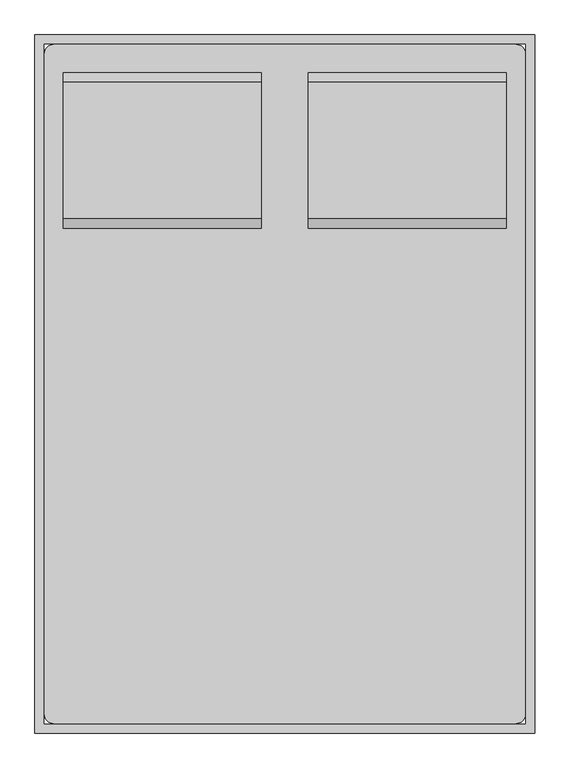
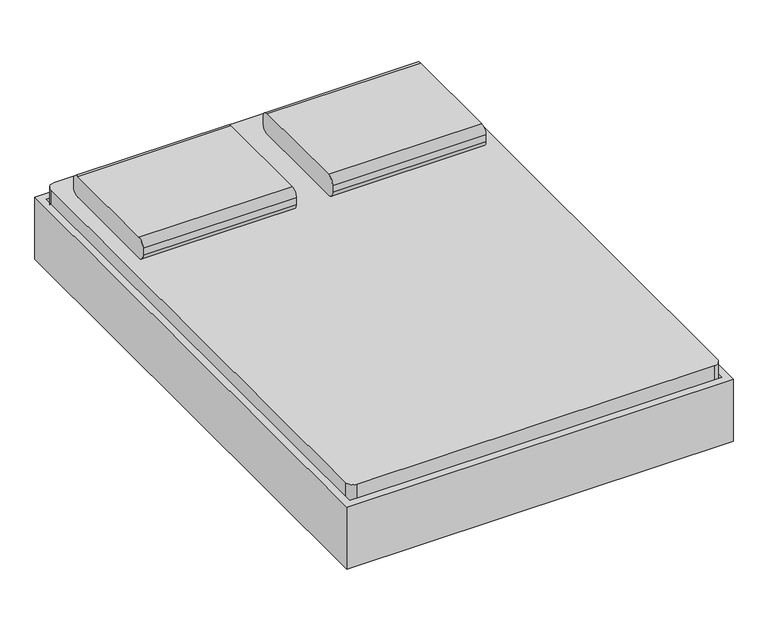
"""IFC4 building model written with IfcOpenShell, lengths in millimetres: furniture geometry, Cama-Caixa : 1346 x 1880 mm - Casal."""

from ifc_helpers import new_model, si_unit, point, frame, frame_2d, origin, place, context, project, spatial, polyline, circle_curve, trimmed, segment, composite_curve, outline, extrude, source, transform, mapped, element, save
from ifc_brep_helpers import plane_surface, cylinder_surface, revolved_surface, advanced_brep


def furniture_b32eb57e(model_context):
    return source(origin(), model_context, "Body", "SolidModel", [
        extrude(outline(composite_curve([segment(polyline([(578.5704918, 406.4), (210.2704918, 406.4)]), True, "CONTINUOUS"), segment(trimmed(circle_curve(frame_2d((210.2704918, 431.8)), 25.4), [point((210.2704918, 406.4))], [point((184.8704918, 431.8))], False, "CARTESIAN"), True, "CONTINUOUS"), segment(polyline([(184.8704918, 431.8), (184.8704918, 457.2)]), True, "CONTINUOUS"), segment(trimmed(circle_curve(frame_2d((210.2704918, 457.2)), 25.4), [point((184.8704918, 457.2))], [point((210.2704918, 482.6))], False, "CARTESIAN"), True, "CONTINUOUS"), segment(polyline([(210.2704918, 482.6), (578.5704918, 482.6)]), True, "CONTINUOUS"), segment(trimmed(circle_curve(frame_2d((578.5704918, 457.2)), 25.4), [point((578.5704918, 482.6))], [point((603.9704918, 457.2))], False, "CARTESIAN"), True, "CONTINUOUS"), segment(polyline([(603.9704918, 457.2), (603.9704918, 431.8)]), True, "CONTINUOUS"), segment(trimmed(circle_curve(frame_2d((578.5704918, 431.8)), 25.4), [point((603.9704918, 431.8))], [point((578.5704918, 406.4))], False, "CARTESIAN"), True, "CONTINUOUS")], self_intersect=False)), frame((402.652459, 0.0, 0.0), z_axis=(1.0, 0.0, 0.0), x_axis=(0.0, 1.0, 0.0)), (0.0, 0.0, 1.0), 533.3),
        extrude(outline(composite_curve([segment(polyline([(578.5704918, 406.4), (210.2704918, 406.4)]), True, "CONTINUOUS"), segment(trimmed(circle_curve(frame_2d((210.2704918, 431.8)), 25.4), [point((210.2704918, 406.4))], [point((184.8704918, 431.8))], False, "CARTESIAN"), True, "CONTINUOUS"), segment(polyline([(184.8704918, 431.8), (184.8704918, 457.2)]), True, "CONTINUOUS"), segment(trimmed(circle_curve(frame_2d((210.2704918, 457.2)), 25.4), [point((184.8704918, 457.2))], [point((210.2704918, 482.6))], False, "CARTESIAN"), True, "CONTINUOUS"), segment(polyline([(210.2704918, 482.6), (578.5704918, 482.6)]), True, "CONTINUOUS"), segment(trimmed(circle_curve(frame_2d((578.5704918, 457.2)), 25.4), [point((578.5704918, 482.6))], [point((603.9704918, 457.2))], False, "CARTESIAN"), True, "CONTINUOUS"), segment(polyline([(603.9704918, 457.2), (603.9704918, 431.8)]), True, "CONTINUOUS"), segment(trimmed(circle_curve(frame_2d((578.5704918, 431.8)), 25.4), [point((603.9704918, 431.8))], [point((578.5704918, 406.4))], False, "CARTESIAN"), True, "CONTINUOUS")], self_intersect=False)), frame((-257.647541, 0.0, 0.0), z_axis=(1.0, 0.0, 0.0), x_axis=(0.0, 1.0, 0.0)), (0.0, 0.0, 1.0), 533.3),
        advanced_brep(
        [(-308.1231784, 451.5704918, 177.8), (-308.1231784, 375.3704918, 177.8), (-308.1231784, 375.3704918, 196.85), (-308.1231784, 451.5704918, 196.85), (-257.3231784, 451.5704918, 177.8), (-257.3231784, 375.3704918, 177.8), (-245.1869899, 375.3704918, 196.85), (-245.1869899, 451.5704918, 196.85), (-181.2523099, 451.5704918, 14.6654962), (-181.2523099, 375.3704918, 14.6654962), (-163.9871466, 375.3704918, 22.716374), (-163.9871466, 451.5704918, 22.716374), (-158.2320921, 375.3704918, 0.0), (-158.2320921, 451.5704918, 0.0), (-158.2320921, 375.3704918, 19.05), (-158.2320921, 451.5704918, 19.05), (-79.6195862, 451.5704918, 0.0), (-79.6195862, 375.3704918, 0.0), (-79.6195862, 375.3704918, 19.05), (-79.6195862, 451.5704918, 19.05), (-66.9195862, 375.3704918, 3.4029547), (-66.9195862, 451.5704918, 3.4029547), (-76.4445862, 375.3704918, 19.9007387), (-76.4445862, 451.5704918, 19.9007387), (-6.822541, 451.5704918, 38.1), (-6.822541, 375.3704918, 38.1), (-11.9269731, 375.3704918, 57.15), (-11.9269731, 451.5704918, 57.15), (685.4518216, 451.5704918, 38.1), (685.4518216, 375.3704918, 38.1), (690.5562537, 375.3704918, 57.15), (690.5562537, 451.5704918, 57.15), (745.5488669, 451.5704918, 3.4029547), (745.5488669, 375.3704918, 3.4029547), (755.0738669, 375.3704918, 19.9007387), (755.0738669, 451.5704918, 19.9007387), (758.2488669, 375.3704918, 0.0), (758.2488669, 451.5704918, 0.0), (758.2488669, 375.3704918, 19.05), (758.2488669, 451.5704918, 19.05), (836.8613728, 451.5704918, 0.0), (836.8613728, 375.3704918, 0.0), (836.8613728, 375.3704918, 19.05), (836.8613728, 451.5704918, 19.05), (859.8815906, 375.3704918, 14.6654962), (859.8815906, 451.5704918, 14.6654962), (842.6164272, 375.3704918, 22.716374), (842.6164272, 451.5704918, 22.716374), (935.952459, 451.5704918, 177.8), (935.952459, 375.3704918, 177.8), (923.8162705, 375.3704918, 196.85), (923.8162705, 451.5704918, 196.85), (986.752459, 451.5704918, 177.8), (986.752459, 451.5704918, 196.85), (986.752459, 375.3704918, 196.85), (986.752459, 375.3704918, 177.8)],
        [
            (0, 1),
            (1, 2),
            (2, 3),
            (3, 0),
            (0, 4),
            (4, 5),
            (5, 1),
            (5, 6),
            (6, 2),
            (6, 7),
            (7, 3),
            (7, 4),
            (4, 8),
            (8, 9),
            (9, 5),
            (9, 10),
            (10, 6),
            (10, 11),
            (11, 7),
            (11, 8),
            (12, 9, circle_curve(frame((-158.2320921, 375.3704918, 25.4), z_axis=(0.0, 1.0, 0.0), x_axis=(-0.906307787036649, 0.0, -0.4226182617407015)), 25.4)),
            (8, 13, circle_curve(frame((-158.2320921, 451.5704918, 25.4), z_axis=(0.0, -1.0, 0.0), x_axis=(-0.906307787036649, 0.0, -0.4226182617407015)), 25.4)),
            (13, 12),
            (14, 10, circle_curve(frame((-158.2320921, 375.3704918, 25.4), z_axis=(0.0, 1.0, 0.0), x_axis=(-0.906307787036649, 0.0, -0.4226182617407015)), 6.35)),
            (12, 14),
            (15, 11, circle_curve(frame((-158.2320921, 451.5704918, 25.4), z_axis=(0.0, 1.0, 0.0), x_axis=(-0.906307787036649, 0.0, -0.4226182617407015)), 6.35)),
            (14, 15),
            (15, 13),
            (13, 16),
            (16, 17),
            (17, 12),
            (17, 18),
            (18, 14),
            (18, 19),
            (19, 15),
            (19, 16),
            (20, 17, circle_curve(frame((-79.6195862, 375.3704918, 25.4), z_axis=(0.0, 1.0, 0.0), x_axis=(0.0, 0.0, -1.0)), 25.4)),
            (16, 21, circle_curve(frame((-79.6195862, 451.5704918, 25.4), z_axis=(0.0, -1.0, 0.0), x_axis=(0.0, 0.0, -1.0)), 25.4)),
            (21, 20),
            (22, 18, circle_curve(frame((-79.6195862, 375.3704918, 25.4), z_axis=(0.0, 1.0, 0.0), x_axis=(0.0, 0.0, -1.0)), 6.35)),
            (20, 22),
            (23, 19, circle_curve(frame((-79.6195862, 451.5704918, 25.4), z_axis=(0.0, 1.0, 0.0), x_axis=(0.0, 0.0, -1.0)), 6.35)),
            (22, 23),
            (23, 21),
            (21, 24),
            (24, 25),
            (25, 20),
            (25, 26),
            (26, 22),
            (26, 27),
            (27, 23),
            (27, 24),
            (24, 28),
            (28, 29),
            (29, 25),
            (29, 30),
            (30, 26),
            (30, 31),
            (31, 27),
            (31, 28),
            (28, 32),
            (32, 33),
            (33, 29),
            (33, 34),
            (34, 30),
            (34, 35),
            (35, 31),
            (35, 32),
            (36, 33, circle_curve(frame((758.2488669, 375.3704918, 25.4), z_axis=(0.0, 1.0, 0.0), x_axis=(-0.5000000000000463, 0.0, -0.8660254037844118)), 25.4)),
            (32, 37, circle_curve(frame((758.2488669, 451.5704918, 25.4), z_axis=(0.0, -1.0, 0.0), x_axis=(-0.5000000000000463, 0.0, -0.8660254037844118)), 25.4)),
            (37, 36),
            (38, 34, circle_curve(frame((758.2488669, 375.3704918, 25.4), z_axis=(0.0, 1.0, 0.0), x_axis=(-0.5000000000000463, 0.0, -0.8660254037844118)), 6.35)),
            (36, 38),
            (39, 35, circle_curve(frame((758.2488669, 451.5704918, 25.4), z_axis=(0.0, 1.0, 0.0), x_axis=(-0.5000000000000463, 0.0, -0.8660254037844118)), 6.35)),
            (38, 39),
            (39, 37),
            (37, 40),
            (40, 41),
            (41, 36),
            (41, 42),
            (42, 38),
            (42, 43),
            (43, 39),
            (43, 40),
            (44, 41, circle_curve(frame((836.8613728, 375.3704918, 25.4), z_axis=(0.0, 1.0, 0.0), x_axis=(0.0, 0.0, -1.0)), 25.4)),
            (40, 45, circle_curve(frame((836.8613728, 451.5704918, 25.4), z_axis=(0.0, -1.0, 0.0), x_axis=(0.0, 0.0, -1.0)), 25.4)),
            (45, 44),
            (46, 42, circle_curve(frame((836.8613728, 375.3704918, 25.4), z_axis=(0.0, 1.0, 0.0), x_axis=(0.0, 0.0, -1.0)), 6.35)),
            (44, 46),
            (47, 43, circle_curve(frame((836.8613728, 451.5704918, 25.4), z_axis=(0.0, 1.0, 0.0), x_axis=(0.0, 0.0, -1.0)), 6.35)),
            (46, 47),
            (47, 45),
            (45, 48),
            (48, 49),
            (49, 44),
            (49, 50),
            (50, 46),
            (50, 51),
            (51, 47),
            (51, 48),
            (52, 53),
            (53, 54),
            (54, 55),
            (55, 52),
            (48, 52),
            (55, 49),
            (54, 50),
            (53, 51),
        ],
        [
            plane_surface(frame((-308.1231784, 705.5704918, -152.9490627), z_axis=(-1.0, 0.0, 0.0), x_axis=(0.0, 1.0, 0.0))),
            plane_surface(frame((-308.1231784, 451.5704918, 177.8), z_axis=(0.0, 0.0, -1.0), x_axis=(1.0, 0.0, 0.0))),
            plane_surface(frame((-308.1231784, 375.3704918, 177.8), z_axis=(0.0, -1.0, 0.0), x_axis=(1.0, 0.0, 0.0))),
            plane_surface(frame((-308.1231784, 375.3704918, 196.85), z_axis=(0.0, 0.0, 1.0), x_axis=(1.0, 0.0, 0.0))),
            plane_surface(frame((-308.1231784, 451.5704918, 196.85), z_axis=(0.0, 1.0, 0.0), x_axis=(1.0, 0.0, 0.0))),
            plane_surface(frame((-257.3231784, 451.5704918, 177.8), z_axis=(-0.9063077870366486, 0.0, -0.4226182617407026), x_axis=(0.4226182617407026, 0.0, -0.9063077870366486))),
            plane_surface(frame((-257.3231784, 375.3704918, 177.8), z_axis=(0.0, -1.0000000000000002, 0.0), x_axis=(0.4226182617407026, 0.0, -0.9063077870366486))),
            plane_surface(frame((-245.1869899, 375.3704918, 196.85), z_axis=(0.9063077870366487, 0.0, 0.4226182617407023), x_axis=(0.4226182617407023, 0.0, -0.9063077870366487))),
            plane_surface(frame((-245.1869899, 451.5704918, 196.85), z_axis=(0.0, 1.0, 0.0), x_axis=(0.4226182617407027, 0.0, -0.9063077870366485))),
            cylinder_surface(frame((-158.2320921, 705.5704918, 25.4), z_axis=(0.0, -1.0, 0.0), x_axis=(-0.906307787036649, 0.0, -0.4226182617407015)), 25.4),
            plane_surface(frame((-158.2320921, 375.3704918, 25.4), z_axis=(0.0, -1.0, 0.0), x_axis=(-0.906307787036649, 0.0, -0.4226182617407015))),
            revolved_surface(polyline([(-163.9871465476827, 375.3704918, 22.716374037946544), (-163.9871465476827, 451.5704918, 22.716374037946544)]), (-158.2320921, 705.5704918, 25.4), (0.0, -1.0, 0.0)),
            plane_surface(frame((-158.2320921, 451.5704918, 25.4), z_axis=(0.0, 1.0, 0.0), x_axis=(-0.906307787036649, 0.0, -0.4226182617407015))),
            plane_surface(frame((-158.2320921, 451.5704918, 0.0), z_axis=(0.0, 0.0, -1.0), x_axis=(1.0, 0.0, 0.0))),
            plane_surface(frame((-158.2320921, 375.3704918, 0.0), z_axis=(0.0, -1.0, 0.0), x_axis=(1.0, 0.0, 0.0))),
            plane_surface(frame((-158.2320921, 375.3704918, 19.05), z_axis=(0.0, 0.0, 1.0), x_axis=(1.0, 0.0, 0.0))),
            plane_surface(frame((-158.2320921, 451.5704918, 19.05), z_axis=(0.0, 1.0, 0.0), x_axis=(1.0, 0.0, 0.0))),
            cylinder_surface(frame((-79.6195862, 705.5704918, 25.4), z_axis=(0.0, -1.0, 0.0), x_axis=(0.0, 0.0, -1.0)), 25.4),
            plane_surface(frame((-79.6195862, 375.3704918, 25.4), z_axis=(0.0, -1.0, 0.0), x_axis=(0.0, 0.0, -1.0))),
            revolved_surface(polyline([(-79.6195862, 375.3704918, 19.049999999999997), (-79.6195862, 451.5704918, 19.049999999999997)]), (-79.6195862, 705.5704918, 25.4), (0.0, -1.0, 0.0)),
            plane_surface(frame((-79.6195862, 451.5704918, 25.4), z_axis=(0.0, 1.0, 0.0), x_axis=(0.0, 0.0, -1.0))),
            plane_surface(frame((-66.9195862, 451.5704918, 3.4029547), z_axis=(0.4999999999998744, 0.0, -0.8660254037845112), x_axis=(0.8660254037845112, 0.0, 0.4999999999998744))),
            plane_surface(frame((-66.9195862, 375.3704918, 3.4029547), z_axis=(0.0, -1.0000000000000002, 0.0), x_axis=(0.8660254037845112, 0.0, 0.4999999999998745))),
            plane_surface(frame((-76.4445862, 375.3704918, 19.9007387), z_axis=(-0.4999999999998741, 0.0, 0.8660254037845113), x_axis=(0.8660254037845113, 0.0, 0.4999999999998741))),
            plane_surface(frame((-76.4445862, 451.5704918, 19.9007387), z_axis=(0.0, 1.0, 0.0), x_axis=(0.866025403784511, 0.0, 0.49999999999987477))),
            plane_surface(frame((-6.822541, 451.5704918, 38.1), z_axis=(0.0, 0.0, -1.0), x_axis=(1.0, 0.0, 0.0))),
            plane_surface(frame((-6.822541, 375.3704918, 38.1), z_axis=(0.0, -1.0, 0.0), x_axis=(1.0, 0.0, 0.0))),
            plane_surface(frame((-11.9269731, 375.3704918, 57.15), z_axis=(0.0, 0.0, 1.0), x_axis=(1.0, 0.0, 0.0))),
            plane_surface(frame((-11.9269731, 451.5704918, 57.15), z_axis=(0.0, 1.0, 0.0), x_axis=(1.0, 0.0, 0.0))),
            plane_surface(frame((685.4518216, 451.5704918, 38.1), z_axis=(-0.5000000000000494, 0.0, -0.8660254037844102), x_axis=(0.8660254037844102, 0.0, -0.5000000000000494))),
            plane_surface(frame((685.4518216, 375.3704918, 38.1), z_axis=(0.0, -1.0, 0.0), x_axis=(0.8660254037844112, 0.0, -0.5000000000000476))),
            plane_surface(frame((690.5562537, 375.3704918, 57.15), z_axis=(0.5000000000000488, 0.0, 0.8660254037844105), x_axis=(0.8660254037844105, 0.0, -0.5000000000000488))),
            plane_surface(frame((690.5562537, 451.5704918, 57.15), z_axis=(0.0, 1.0, 0.0), x_axis=(0.8660254037844106, 0.0, -0.5000000000000485))),
            cylinder_surface(frame((758.2488669, 705.5704918, 25.4), z_axis=(0.0, -1.0, 0.0), x_axis=(-0.5000000000000463, 0.0, -0.8660254037844118)), 25.4),
            plane_surface(frame((758.2488669, 375.3704918, 25.4), z_axis=(0.0, -1.0000000000000002, 0.0), x_axis=(-0.5000000000000464, 0.0, -0.866025403784412))),
            revolved_surface(polyline([(755.0738668999998, 375.3704918, 19.90073868596898), (755.0738668999998, 451.5704918, 19.90073868596898)]), (758.2488669, 705.5704918, 25.4), (0.0, -1.0, 0.0)),
            plane_surface(frame((758.2488669, 451.5704918, 25.4), z_axis=(0.0, 1.0000000000000002, 0.0), x_axis=(-0.5000000000000464, 0.0, -0.866025403784412))),
            plane_surface(frame((758.2488669, 451.5704918, 0.0), z_axis=(0.0, 0.0, -1.0), x_axis=(1.0, 0.0, 0.0))),
            plane_surface(frame((758.2488669, 375.3704918, 0.0), z_axis=(0.0, -1.0, 0.0), x_axis=(1.0, 0.0, 0.0))),
            plane_surface(frame((758.2488669, 375.3704918, 19.05), z_axis=(0.0, 0.0, 1.0), x_axis=(1.0, 0.0, 0.0))),
            plane_surface(frame((758.2488669, 451.5704918, 19.05), z_axis=(0.0, 1.0, 0.0), x_axis=(1.0, 0.0, 0.0))),
            cylinder_surface(frame((836.8613728, 705.5704918, 25.4), z_axis=(0.0, -1.0, 0.0), x_axis=(0.0, 0.0, -1.0)), 25.4),
            plane_surface(frame((836.8613728, 375.3704918, 25.4), z_axis=(0.0, -1.0, 0.0), x_axis=(0.0, 0.0, -1.0))),
            revolved_surface(polyline([(836.8613728, 375.3704918, 19.049999999999997), (836.8613728, 451.5704918, 19.049999999999997)]), (836.8613728, 705.5704918, 25.4), (0.0, -1.0, 0.0)),
            plane_surface(frame((836.8613728, 451.5704918, 25.4), z_axis=(0.0, 1.0, 0.0), x_axis=(0.0, 0.0, -1.0))),
            plane_surface(frame((859.8815906, 451.5704918, 14.6654962), z_axis=(0.90630778703668, 0.0, -0.422618261740635), x_axis=(0.422618261740635, 0.0, 0.90630778703668))),
            plane_surface(frame((859.8815906, 375.3704918, 14.6654962), z_axis=(0.0, -1.0000000000000002, 0.0), x_axis=(0.4226182617406349, 0.0, 0.9063077870366801))),
            plane_surface(frame((842.6164272, 375.3704918, 22.716374), z_axis=(-0.9063077870366805, 0.0, 0.4226182617406341), x_axis=(0.4226182617406341, 0.0, 0.9063077870366805))),
            plane_surface(frame((842.6164272, 451.5704918, 22.716374), z_axis=(0.0, 1.0, 0.0), x_axis=(0.42261826174063455, 0.0, 0.9063077870366802))),
            plane_surface(frame((986.752459, 705.5704918, -152.9490627), z_axis=(1.0, 0.0, 0.0), x_axis=(0.0, 1.0, 0.0))),
            plane_surface(frame((935.952459, 451.5704918, 177.8), z_axis=(0.0, 0.0, -1.0), x_axis=(1.0, 0.0, 0.0))),
            plane_surface(frame((935.952459, 375.3704918, 177.8), z_axis=(0.0, -1.0, 0.0), x_axis=(1.0, 0.0, 0.0))),
            plane_surface(frame((923.8162705, 375.3704918, 196.85), z_axis=(0.0, 0.0, 1.0), x_axis=(1.0, 0.0, 0.0))),
            plane_surface(frame((923.8162705, 451.5704918, 196.85), z_axis=(0.0, 1.0, 0.0), x_axis=(1.0, 0.0, 0.0))),
        ],
        [
            (0, [[1, 2, 3, 4]]),
            (1, [[-1, 5, 6, 7]]),
            (2, [[-2, -7, 8, 9]]),
            (3, [[-3, -9, 10, 11]]),
            (4, [[-4, -11, 12, -5]]),
            (5, [[-6, 13, 14, 15]]),
            (6, [[-8, -15, 16, 17]]),
            (7, [[-10, -17, 18, 19]]),
            (8, [[-12, -19, 20, -13]]),
            (9, [[21, -14, 22, 23]]),
            (10, [[24, -16, -21, 25]]),
            (11, [[26, -18, -24, 27]]),
            (12, [[-22, -20, -26, 28]]),
            (13, [[-23, 29, 30, 31]]),
            (14, [[-25, -31, 32, 33]]),
            (15, [[-27, -33, 34, 35]]),
            (16, [[-28, -35, 36, -29]]),
            (17, [[37, -30, 38, 39]]),
            (18, [[40, -32, -37, 41]]),
            (19, [[42, -34, -40, 43]]),
            (20, [[-38, -36, -42, 44]]),
            (21, [[-39, 45, 46, 47]]),
            (22, [[-41, -47, 48, 49]]),
            (23, [[-43, -49, 50, 51]]),
            (24, [[-44, -51, 52, -45]]),
            (25, [[-46, 53, 54, 55]]),
            (26, [[-48, -55, 56, 57]]),
            (27, [[-50, -57, 58, 59]]),
            (28, [[-52, -59, 60, -53]]),
            (29, [[-54, 61, 62, 63]]),
            (30, [[-56, -63, 64, 65]]),
            (31, [[-58, -65, 66, 67]]),
            (32, [[-60, -67, 68, -61]]),
            (33, [[69, -62, 70, 71]]),
            (34, [[72, -64, -69, 73]]),
            (35, [[74, -66, -72, 75]]),
            (36, [[-70, -68, -74, 76]]),
            (37, [[-71, 77, 78, 79]]),
            (38, [[-73, -79, 80, 81]]),
            (39, [[-75, -81, 82, 83]]),
            (40, [[-76, -83, 84, -77]]),
            (41, [[85, -78, 86, 87]]),
            (42, [[88, -80, -85, 89]]),
            (43, [[90, -82, -88, 91]]),
            (44, [[-86, -84, -90, 92]]),
            (45, [[-87, 93, 94, 95]]),
            (46, [[-89, -95, 96, 97]]),
            (47, [[-91, -97, 98, 99]]),
            (48, [[-92, -99, 100, -93]]),
            (49, [[101, 102, 103, 104]]),
            (50, [[-94, 105, -104, 106]]),
            (51, [[-96, -106, -103, 107]]),
            (52, [[-98, -107, -102, 108]]),
            (53, [[-100, -108, -101, -105]]),
        ],
    ),
        extrude(outline(composite_curve([segment(polyline([(-283.047541, 680.1704918), (961.352459, 680.1704918)]), True, "CONTINUOUS"), segment(trimmed(circle_curve(frame_2d((961.352459, 654.7704918)), 25.4), [point((961.352459, 680.1704918))], [point((986.752459, 654.7704918))], False, "CARTESIAN"), True, "CONTINUOUS"), segment(polyline([(986.752459, 654.7704918), (986.752459, -1123.6295082)]), True, "CONTINUOUS"), segment(trimmed(circle_curve(frame_2d((961.352459, -1123.6295082)), 25.4), [point((986.752459, -1123.6295082))], [point((961.352459, -1149.0295082))], False, "CARTESIAN"), True, "CONTINUOUS"), segment(polyline([(961.352459, -1149.0295082), (-283.047541, -1149.0295082)]), True, "CONTINUOUS"), segment(trimmed(circle_curve(frame_2d((-283.047541, -1123.6295082)), 25.4), [point((-283.047541, -1149.0295082))], [point((-308.447541, -1123.6295082))], False, "CARTESIAN"), True, "CONTINUOUS"), segment(polyline([(-308.447541, -1123.6295082), (-308.447541, 654.7704918)]), True, "CONTINUOUS"), segment(trimmed(circle_curve(frame_2d((-283.047541, 654.7704918)), 25.4), [point((-308.447541, 654.7704918))], [point((-283.047541, 680.1704918))], False, "CARTESIAN"), True, "CONTINUOUS")], self_intersect=False)), frame((0.0, 0.0, 203.2), z_axis=(0.0, 0.0, 1.0), x_axis=(1.0, 0.0, 0.0)), (0.0, 0.0, 1.0), 203.2),
        advanced_brep(
        [(-308.447541, -869.6295082, 196.85), (-308.447541, -869.6295082, 177.8), (-308.447541, -945.8295082, 177.8), (-308.447541, -945.8295082, 196.85), (-245.5113525, -869.6295082, 196.85), (-257.647541, -869.6295082, 177.8), (-257.647541, -945.8295082, 177.8), (-245.5113525, -945.8295082, 196.85), (-164.3115092, -869.6295082, 22.716374), (-181.5766725, -869.6295082, 14.6654962), (-181.5766725, -945.8295082, 14.6654962), (-164.3115092, -945.8295082, 22.716374), (-158.5564547, -869.6295082, 0.0), (-158.5564547, -869.6295082, 19.05), (-158.5564547, -945.8295082, 0.0), (-158.5564547, -945.8295082, 19.05), (-79.9439489, -869.6295082, 19.05), (-79.9439489, -869.6295082, 0.0), (-79.9439489, -945.8295082, 0.0), (-79.9439489, -945.8295082, 19.05), (-67.2439489, -869.6295082, 3.4029547), (-76.7689489, -869.6295082, 19.9007387), (-67.2439489, -945.8295082, 3.4029547), (-76.7689489, -945.8295082, 19.9007387), (-12.2513357, -869.6295082, 57.15), (-7.1469036, -869.6295082, 38.1), (-7.1469036, -945.8295082, 38.1), (-12.2513357, -945.8295082, 57.15), (690.5562537, -869.6295082, 57.15), (685.4518216, -869.6295082, 38.1), (685.4518216, -945.8295082, 38.1), (690.5562537, -945.8295082, 57.15), (755.0738669, -869.6295082, 19.9007387), (745.5488669, -869.6295082, 3.4029547), (745.5488669, -945.8295082, 3.4029547), (755.0738669, -945.8295082, 19.9007387), (758.2488669, -869.6295082, 0.0), (758.2488669, -869.6295082, 19.05), (758.2488669, -945.8295082, 0.0), (758.2488669, -945.8295082, 19.05), (836.8613728, -869.6295082, 19.05), (836.8613728, -869.6295082, 0.0), (836.8613728, -945.8295082, 0.0), (836.8613728, -945.8295082, 19.05), (859.8815906, -869.6295082, 14.6654962), (842.6164272, -869.6295082, 22.716374), (859.8815906, -945.8295082, 14.6654962), (842.6164272, -945.8295082, 22.716374), (923.8162705, -869.6295082, 196.85), (935.952459, -869.6295082, 177.8), (935.952459, -945.8295082, 177.8), (923.8162705, -945.8295082, 196.85), (986.752459, -869.6295082, 196.85), (986.752459, -945.8295082, 196.85), (986.752459, -945.8295082, 177.8), (986.752459, -869.6295082, 177.8)],
        [
            (0, 1),
            (1, 2),
            (2, 3),
            (3, 0),
            (0, 4),
            (4, 5),
            (5, 1),
            (5, 6),
            (6, 2),
            (6, 7),
            (7, 3),
            (7, 4),
            (4, 8),
            (8, 9),
            (9, 5),
            (9, 10),
            (10, 6),
            (10, 11),
            (11, 7),
            (11, 8),
            (12, 9, circle_curve(frame((-158.5564547, -869.6295082, 25.4), z_axis=(0.0, 1.0, 0.0), x_axis=(-0.9063077870366625, 0.0, -0.4226182617406725)), 25.4)),
            (8, 13, circle_curve(frame((-158.5564547, -869.6295082, 25.4), z_axis=(0.0, -1.0, 0.0), x_axis=(-0.9063077870366625, 0.0, -0.4226182617406725)), 6.35)),
            (13, 12),
            (14, 10, circle_curve(frame((-158.5564547, -945.8295082, 25.4), z_axis=(0.0, 1.0, 0.0), x_axis=(-0.9063077870366625, 0.0, -0.4226182617406725)), 25.4)),
            (12, 14),
            (15, 11, circle_curve(frame((-158.5564547, -945.8295082, 25.4), z_axis=(0.0, 1.0, 0.0), x_axis=(-0.9063077870366625, 0.0, -0.4226182617406725)), 6.35)),
            (14, 15),
            (15, 13),
            (13, 16),
            (16, 17),
            (17, 12),
            (17, 18),
            (18, 14),
            (18, 19),
            (19, 15),
            (19, 16),
            (20, 17, circle_curve(frame((-79.9439489, -869.6295082, 25.4), z_axis=(0.0, 1.0, 0.0), x_axis=(0.0, 0.0, -1.0)), 25.4)),
            (16, 21, circle_curve(frame((-79.9439489, -869.6295082, 25.4), z_axis=(0.0, -1.0, 0.0), x_axis=(0.0, 0.0, -1.0)), 6.35)),
            (21, 20),
            (22, 18, circle_curve(frame((-79.9439489, -945.8295082, 25.4), z_axis=(0.0, 1.0, 0.0), x_axis=(0.0, 0.0, -1.0)), 25.4)),
            (20, 22),
            (23, 19, circle_curve(frame((-79.9439489, -945.8295082, 25.4), z_axis=(0.0, 1.0, 0.0), x_axis=(0.0, 0.0, -1.0)), 6.35)),
            (22, 23),
            (23, 21),
            (21, 24),
            (24, 25),
            (25, 20),
            (25, 26),
            (26, 22),
            (26, 27),
            (27, 23),
            (27, 24),
            (24, 28),
            (28, 29),
            (29, 25),
            (29, 30),
            (30, 26),
            (30, 31),
            (31, 27),
            (31, 28),
            (28, 32),
            (32, 33),
            (33, 29),
            (33, 34),
            (34, 30),
            (34, 35),
            (35, 31),
            (35, 32),
            (36, 33, circle_curve(frame((758.2488669, -869.6295082, 25.4), z_axis=(0.0, 1.0, 0.0), x_axis=(-0.5000000000000528, 0.0, -0.8660254037844081)), 25.4)),
            (32, 37, circle_curve(frame((758.2488669, -869.6295082, 25.4), z_axis=(0.0, -1.0, 0.0), x_axis=(-0.5000000000000528, 0.0, -0.8660254037844081)), 6.35)),
            (37, 36),
            (38, 34, circle_curve(frame((758.2488669, -945.8295082, 25.4), z_axis=(0.0, 1.0, 0.0), x_axis=(-0.5000000000000528, 0.0, -0.8660254037844081)), 25.4)),
            (36, 38),
            (39, 35, circle_curve(frame((758.2488669, -945.8295082, 25.4), z_axis=(0.0, 1.0, 0.0), x_axis=(-0.5000000000000528, 0.0, -0.8660254037844081)), 6.35)),
            (38, 39),
            (39, 37),
            (37, 40),
            (40, 41),
            (41, 36),
            (41, 42),
            (42, 38),
            (42, 43),
            (43, 39),
            (43, 40),
            (44, 41, circle_curve(frame((836.8613728, -869.6295082, 25.4), z_axis=(0.0, 1.0, 0.0), x_axis=(0.0, 0.0, -1.0)), 25.4)),
            (40, 45, circle_curve(frame((836.8613728, -869.6295082, 25.4), z_axis=(0.0, -1.0, 0.0), x_axis=(0.0, 0.0, -1.0)), 6.35)),
            (45, 44),
            (46, 42, circle_curve(frame((836.8613728, -945.8295082, 25.4), z_axis=(0.0, 1.0, 0.0), x_axis=(0.0, 0.0, -1.0)), 25.4)),
            (44, 46),
            (47, 43, circle_curve(frame((836.8613728, -945.8295082, 25.4), z_axis=(0.0, 1.0, 0.0), x_axis=(0.0, 0.0, -1.0)), 6.35)),
            (46, 47),
            (47, 45),
            (45, 48),
            (48, 49),
            (49, 44),
            (49, 50),
            (50, 46),
            (50, 51),
            (51, 47),
            (51, 48),
            (52, 53),
            (53, 54),
            (54, 55),
            (55, 52),
            (48, 52),
            (55, 49),
            (54, 50),
            (53, 51),
        ],
        [
            plane_surface(frame((-308.447541, -1174.4295082, -127.5947323), z_axis=(-1.0, 0.0, 0.0), x_axis=(0.0, 1.0, 0.0))),
            plane_surface(frame((-308.447541, -869.6295082, 196.85), z_axis=(0.0, 1.0, 0.0), x_axis=(1.0, 0.0, 0.0))),
            plane_surface(frame((-308.447541, -869.6295082, 177.8), z_axis=(0.0, 0.0, -1.0), x_axis=(1.0, 0.0, 0.0))),
            plane_surface(frame((-308.447541, -945.8295082, 177.8), z_axis=(0.0, -1.0, 0.0), x_axis=(1.0, 0.0, 0.0))),
            plane_surface(frame((-308.447541, -945.8295082, 196.85), z_axis=(0.0, 0.0, 1.0), x_axis=(1.0, 0.0, 0.0))),
            plane_surface(frame((-245.5113525, -869.6295082, 196.85), z_axis=(0.0, 1.0, 0.0), x_axis=(0.4226182617406714, 0.0, -0.906307787036663))),
            plane_surface(frame((-257.647541, -869.6295082, 177.8), z_axis=(-0.9063077870366631, 0.0, -0.42261826174067146), x_axis=(0.42261826174067146, 0.0, -0.9063077870366631))),
            plane_surface(frame((-257.647541, -945.8295082, 177.8), z_axis=(0.0, -1.0000000000000002, 0.0), x_axis=(0.4226182617406716, 0.0, -0.906307787036663))),
            plane_surface(frame((-245.5113525, -945.8295082, 196.85), z_axis=(0.906307787036663, 0.0, 0.4226182617406716), x_axis=(0.4226182617406716, 0.0, -0.906307787036663))),
            plane_surface(frame((-158.5564547, -869.6295082, 25.4), z_axis=(0.0, 1.0, 0.0), x_axis=(-0.9063077870366625, 0.0, -0.4226182617406725))),
            cylinder_surface(frame((-158.5564547, -1174.4295082, 25.4), z_axis=(0.0, -1.0, 0.0), x_axis=(-0.9063077870366625, 0.0, -0.4226182617406725)), 25.4),
            plane_surface(frame((-158.5564547, -945.8295082, 25.4), z_axis=(0.0, -1.0, 0.0), x_axis=(-0.9063077870366625, 0.0, -0.4226182617406725))),
            revolved_surface(polyline([(-164.31150914768278, -945.8295082, 22.71637403794673), (-164.31150914768278, -869.6295082, 22.71637403794673)]), (-158.5564547, -1174.4295082, 25.4), (0.0, -1.0, 0.0)),
            plane_surface(frame((-158.5564547, -869.6295082, 19.05), z_axis=(0.0, 1.0, 0.0), x_axis=(1.0, 0.0, 0.0))),
            plane_surface(frame((-158.5564547, -869.6295082, 0.0), z_axis=(0.0, 0.0, -1.0), x_axis=(1.0, 0.0, 0.0))),
            plane_surface(frame((-158.5564547, -945.8295082, 0.0), z_axis=(0.0, -1.0, 0.0), x_axis=(1.0, 0.0, 0.0))),
            plane_surface(frame((-158.5564547, -945.8295082, 19.05), z_axis=(0.0, 0.0, 1.0), x_axis=(1.0, 0.0, 0.0))),
            plane_surface(frame((-79.9439489, -869.6295082, 25.4), z_axis=(0.0, 1.0, 0.0), x_axis=(0.0, 0.0, -1.0))),
            cylinder_surface(frame((-79.9439489, -1174.4295082, 25.4), z_axis=(0.0, -1.0, 0.0), x_axis=(0.0, 0.0, -1.0)), 25.4),
            plane_surface(frame((-79.9439489, -945.8295082, 25.4), z_axis=(0.0, -1.0, 0.0), x_axis=(0.0, 0.0, -1.0))),
            revolved_surface(polyline([(-79.9439489, -945.8295082, 19.049999999999997), (-79.9439489, -869.6295082, 19.049999999999997)]), (-79.9439489, -1174.4295082, 25.4), (0.0, -1.0, 0.0)),
            plane_surface(frame((-76.7689489, -869.6295082, 19.9007387), z_axis=(0.0, 1.0000000000000002, 0.0), x_axis=(0.8660254037844788, 0.0, 0.49999999999993067))),
            plane_surface(frame((-67.2439489, -869.6295082, 3.4029547), z_axis=(0.49999999999993067, 0.0, -0.8660254037844787), x_axis=(0.8660254037844787, 0.0, 0.49999999999993067))),
            plane_surface(frame((-67.2439489, -945.8295082, 3.4029547), z_axis=(0.0, -1.0, 0.0), x_axis=(0.8660254037844782, 0.0, 0.4999999999999315))),
            plane_surface(frame((-76.7689489, -945.8295082, 19.9007387), z_axis=(-0.49999999999993044, 0.0, 0.8660254037844789), x_axis=(0.8660254037844789, 0.0, 0.49999999999993044))),
            plane_surface(frame((-12.2513357, -869.6295082, 57.15), z_axis=(0.0, 1.0, 0.0), x_axis=(1.0, 0.0, 0.0))),
            plane_surface(frame((-7.1469036, -869.6295082, 38.1), z_axis=(0.0, 0.0, -1.0), x_axis=(1.0, 0.0, 0.0))),
            plane_surface(frame((-7.1469036, -945.8295082, 38.1), z_axis=(0.0, -1.0, 0.0), x_axis=(1.0, 0.0, 0.0))),
            plane_surface(frame((-12.2513357, -945.8295082, 57.15), z_axis=(0.0, 0.0, 1.0), x_axis=(1.0, 0.0, 0.0))),
            plane_surface(frame((690.5562537, -869.6295082, 57.15), z_axis=(0.0, 1.0, 0.0), x_axis=(0.8660254037844087, 0.0, -0.5000000000000518))),
            plane_surface(frame((685.4518216, -869.6295082, 38.1), z_axis=(-0.5000000000000513, 0.0, -0.8660254037844092), x_axis=(0.8660254037844092, 0.0, -0.5000000000000513))),
            plane_surface(frame((685.4518216, -945.8295082, 38.1), z_axis=(0.0, -1.0, 0.0), x_axis=(0.8660254037844081, 0.0, -0.5000000000000531))),
            plane_surface(frame((690.5562537, -945.8295082, 57.15), z_axis=(0.5000000000000521, 0.0, 0.8660254037844086), x_axis=(0.8660254037844086, 0.0, -0.5000000000000521))),
            plane_surface(frame((758.2488669, -869.6295082, 25.4), z_axis=(0.0, 1.0000000000000002, 0.0), x_axis=(-0.500000000000053, 0.0, -0.8660254037844082))),
            cylinder_surface(frame((758.2488669, -1174.4295082, 25.4), z_axis=(0.0, -1.0, 0.0), x_axis=(-0.5000000000000528, 0.0, -0.8660254037844081)), 25.4),
            plane_surface(frame((758.2488669, -945.8295082, 25.4), z_axis=(0.0, -1.0000000000000002, 0.0), x_axis=(-0.500000000000053, 0.0, -0.8660254037844082))),
            revolved_surface(polyline([(755.0738668999998, -945.8295082, 19.900738685969007), (755.0738668999998, -869.6295082, 19.900738685969007)]), (758.2488669, -1174.4295082, 25.4), (0.0, -1.0, 0.0)),
            plane_surface(frame((758.2488669, -869.6295082, 19.05), z_axis=(0.0, 1.0, 0.0), x_axis=(1.0, 0.0, 0.0))),
            plane_surface(frame((758.2488669, -869.6295082, 0.0), z_axis=(0.0, 0.0, -1.0), x_axis=(1.0, 0.0, 0.0))),
            plane_surface(frame((758.2488669, -945.8295082, 0.0), z_axis=(0.0, -1.0, 0.0), x_axis=(1.0, 0.0, 0.0))),
            plane_surface(frame((758.2488669, -945.8295082, 19.05), z_axis=(0.0, 0.0, 1.0), x_axis=(1.0, 0.0, 0.0))),
            plane_surface(frame((836.8613728, -869.6295082, 25.4), z_axis=(0.0, 1.0, 0.0), x_axis=(0.0, 0.0, -1.0))),
            cylinder_surface(frame((836.8613728, -1174.4295082, 25.4), z_axis=(0.0, -1.0, 0.0), x_axis=(0.0, 0.0, -1.0)), 25.4),
            plane_surface(frame((836.8613728, -945.8295082, 25.4), z_axis=(0.0, -1.0, 0.0), x_axis=(0.0, 0.0, -1.0))),
            revolved_surface(polyline([(836.8613728, -945.8295082, 19.049999999999997), (836.8613728, -869.6295082, 19.049999999999997)]), (836.8613728, -1174.4295082, 25.4), (0.0, -1.0, 0.0)),
            plane_surface(frame((842.6164272, -869.6295082, 22.716374), z_axis=(0.0, 1.0, 0.0), x_axis=(0.4226182617405387, 0.0, 0.906307787036725))),
            plane_surface(frame((859.8815906, -869.6295082, 14.6654962), z_axis=(0.906307787036725, 0.0, -0.4226182617405386), x_axis=(0.4226182617405386, 0.0, 0.906307787036725))),
            plane_surface(frame((859.8815906, -945.8295082, 14.6654962), z_axis=(0.0, -1.0, 0.0), x_axis=(0.4226182617405387, 0.0, 0.906307787036725))),
            plane_surface(frame((842.6164272, -945.8295082, 22.716374), z_axis=(-0.9063077870367251, 0.0, 0.4226182617405384), x_axis=(0.4226182617405384, 0.0, 0.9063077870367251))),
            plane_surface(frame((986.752459, -1174.4295082, -127.5947323), z_axis=(1.0, 0.0, 0.0), x_axis=(0.0, 1.0, 0.0))),
            plane_surface(frame((923.8162705, -869.6295082, 196.85), z_axis=(0.0, 1.0, 0.0), x_axis=(1.0, 0.0, 0.0))),
            plane_surface(frame((935.952459, -869.6295082, 177.8), z_axis=(0.0, 0.0, -1.0), x_axis=(1.0, 0.0, 0.0))),
            plane_surface(frame((935.952459, -945.8295082, 177.8), z_axis=(0.0, -1.0, 0.0), x_axis=(1.0, 0.0, 0.0))),
            plane_surface(frame((923.8162705, -945.8295082, 196.85), z_axis=(0.0, 0.0, 1.0), x_axis=(1.0, 0.0, 0.0))),
        ],
        [
            (0, [[1, 2, 3, 4]]),
            (1, [[-1, 5, 6, 7]]),
            (2, [[-2, -7, 8, 9]]),
            (3, [[-3, -9, 10, 11]]),
            (4, [[-4, -11, 12, -5]]),
            (5, [[-6, 13, 14, 15]]),
            (6, [[-8, -15, 16, 17]]),
            (7, [[-10, -17, 18, 19]]),
            (8, [[-12, -19, 20, -13]]),
            (9, [[21, -14, 22, 23]]),
            (10, [[24, -16, -21, 25]]),
            (11, [[26, -18, -24, 27]]),
            (12, [[-22, -20, -26, 28]]),
            (13, [[-23, 29, 30, 31]]),
            (14, [[-25, -31, 32, 33]]),
            (15, [[-27, -33, 34, 35]]),
            (16, [[-28, -35, 36, -29]]),
            (17, [[37, -30, 38, 39]]),
            (18, [[40, -32, -37, 41]]),
            (19, [[42, -34, -40, 43]]),
            (20, [[-38, -36, -42, 44]]),
            (21, [[-39, 45, 46, 47]]),
            (22, [[-41, -47, 48, 49]]),
            (23, [[-43, -49, 50, 51]]),
            (24, [[-44, -51, 52, -45]]),
            (25, [[-46, 53, 54, 55]]),
            (26, [[-48, -55, 56, 57]]),
            (27, [[-50, -57, 58, 59]]),
            (28, [[-52, -59, 60, -53]]),
            (29, [[-54, 61, 62, 63]]),
            (30, [[-56, -63, 64, 65]]),
            (31, [[-58, -65, 66, 67]]),
            (32, [[-60, -67, 68, -61]]),
            (33, [[69, -62, 70, 71]]),
            (34, [[72, -64, -69, 73]]),
            (35, [[74, -66, -72, 75]]),
            (36, [[-70, -68, -74, 76]]),
            (37, [[-71, 77, 78, 79]]),
            (38, [[-73, -79, 80, 81]]),
            (39, [[-75, -81, 82, 83]]),
            (40, [[-76, -83, 84, -77]]),
            (41, [[85, -78, 86, 87]]),
            (42, [[88, -80, -85, 89]]),
            (43, [[90, -82, -88, 91]]),
            (44, [[-86, -84, -90, 92]]),
            (45, [[-87, 93, 94, 95]]),
            (46, [[-89, -95, 96, 97]]),
            (47, [[-91, -97, 98, 99]]),
            (48, [[-92, -99, 100, -93]]),
            (49, [[101, 102, 103, 104]]),
            (50, [[-94, 105, -104, 106]]),
            (51, [[-96, -106, -103, 107]]),
            (52, [[-98, -107, -102, 108]]),
            (53, [[-100, -108, -101, -105]]),
        ],
    ),
        extrude(outline(polyline([(1012.152459, 705.5704918), (1012.152459, -1174.4295082), (-333.847541, -1174.4295082), (-333.847541, 705.5704918), (1012.152459, 705.5704918)]), holes=[polyline([(986.752459, 680.1704918), (-308.447541, 680.1704918), (-308.447541, -1149.0295082), (986.752459, -1149.0295082), (986.752459, 680.1704918)])]), frame((0.0, 0.0, 127.0), z_axis=(0.0, 0.0, 1.0), x_axis=(1.0, 0.0, 0.0)), (0.0, 0.0, 1.0), 228.6),
    ])


if __name__ == "__main__":
    model = new_model("IFC4")
    model_context = context("Model", 3, world=origin())
    ifc_project = project(units=[si_unit("LENGTHUNIT", "METRE", prefix="MILLI")], contexts=[model_context])
    site = spatial("IfcSite", under=ifc_project)
    building = spatial("IfcBuilding", under=site)
    placement = place(None, origin())
    furniture_shape = furniture_b32eb57e(model_context)
    element("IfcFurniture", 1, ObjectType="Cama-Caixa : 1346 x 1880 mm - Casal", at=placement, inside=building, context=model_context, shape_type="MappedRepresentation", body=[
        mapped(furniture_shape, transform((0.0, 0.0, 0.0), x_axis=(1.0, 0.0, 0.0), y_axis=(0.0, 1.0, 0.0), z_axis=(0.0, 0.0, 1.0))),
    ])
    save(model, "model.ifc")

# Revit data of these elements
# Type "Cama-Caixa : 1346 x 1880 mm - Casal"
#   Comprimento = 1880 mm
#   Largura = 1346 mm
#   Material da moldura = Bétula
#   Material do colchão = Linho, branco
# Element 1 (IfcFurniture, "Cama-Caixa : 1346 x 1880 mm - Casal")
#   Materials on its faces: "Bétula", "Linho, branco"
# Materials
#   "Bétula": class "Madeira", colour RGB 224 178 126, transparency 0, Description = "Bétula Alleghaniensis", Cost = 0
#   "Linho, branco": class "Tecido", colour RGB 247 247 239, transparency 0, Description = "Linho, branco", Cost = 0
